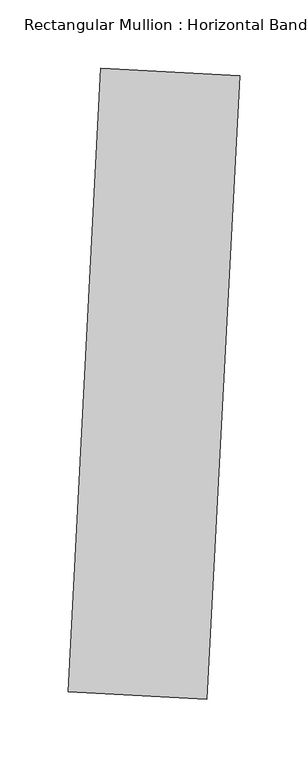
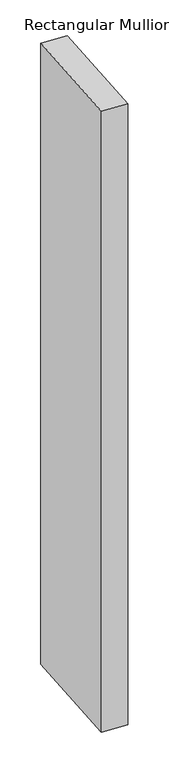
"""IFC4 building model written with IfcOpenShell, lengths in millimetres: member geometry, Rectangular Mullion : Horizontal Band."""

from ifc_helpers import new_model, si_unit, frame, origin, place, context, project, spatial, polyline, outline, extrude, source, transform, mapped, element, save


def rectangular_mullion_horizontal_band_838d4356(model_context):
    return source(origin(), model_context, "Body", "SweptSolid", [
        extrude(outline(polyline([(62.69438, 301.8280451), (38.7663808, -154.7453782), (-62.69438, -149.4280451), (-38.7663808, 307.1453782), (62.69438, 301.8280451)])), frame((0.0, 0.0, -2603.6943143), z_axis=(0.0, 0.0, 1.0), x_axis=(1.0, 0.0, 0.0)), (0.0, 0.0, 1.0), 2603.6943143),
    ])


if __name__ == "__main__":
    model = new_model("IFC4")
    model_context = context("Model", 3, world=origin())
    ifc_project = project(units=[si_unit("LENGTHUNIT", "METRE", prefix="MILLI")], contexts=[model_context])
    site = spatial("IfcSite", under=ifc_project)
    building = spatial("IfcBuilding", under=site)
    placement = place(None, origin())
    rectangular_mullion_horizontal_band_shape = rectangular_mullion_horizontal_band_838d4356(model_context)
    element("IfcMember", 1, ObjectType="Rectangular Mullion : Horizontal Band", at=placement, inside=building, context=model_context, shape_type="MappedRepresentation", body=[
        mapped(rectangular_mullion_horizontal_band_shape, transform((0.0, 0.0, 0.0), x_axis=(1.0, 0.0, 0.0), y_axis=(0.0, 1.0, 0.0), z_axis=(0.0, 0.0, 1.0))),
    ])
    save(model, "model.ifc")

# Revit data of these elements
# Type "Rectangular Mullion : Horizontal Band"
#   built-in parameter 1007351 = 0.25 (stored number, unit not read)
#   built-in parameter 1007304 = 1.5 (stored number, unit not read)
#   built-in parameter 1007301 = 0.166667 (stored number, unit not read)
#   built-in parameter 1007300 = 0.166667 (stored number, unit not read)
# Element 1 (IfcMember, "Rectangular Mullion : Horizontal Band")
#   Materials on its faces: "Aluminum"
# Materials
#   "Aluminum": class "Metal", colour RGB 247 247 247, transparency 0, Description = "Aluminum 6061", Cost = 0
